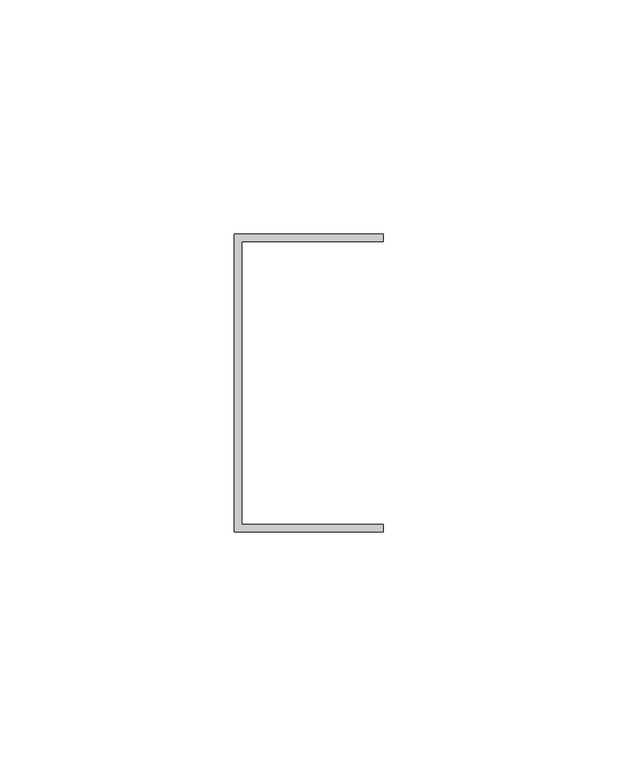
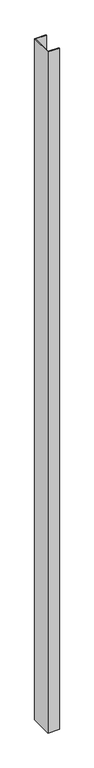
"""IFC4 building model written with IfcOpenShell, lengths in millimetres: proxy geometry, Generic Models 7:Generic Models 1:3:Generic Models 1:3 : Generic Models 7:Generic Models 1:305549:3:Generic Models 1:3:Generic Models 1:3 : Generic Models 7:Generic Models 1:305549:3 : Generic Models 7:Generic Models 1:3:Generic Models 1:3 : Generic Models 7:Generic Models 1:305549:301244:11 : Generic Models 7:Generic Models 1:3:Generic Models 1:3 : Generic Models 7:Generic Models 1:305549:3:Generic Models 1:3:Generic Models 1:3 : Generic Models 7:Generic Models 1:305549:3 : Generic Models 7:Generic Models 1:3:Generic Models 1:3 : Generic Models 7:Generic Models 1:305549:301244:308848."""

from ifc_helpers import new_model, si_unit, frame, origin, place, context, project, spatial, polyline, outline, extrude, source, transform, mapped, element, save


def generic_models_456df3e6(model_context):
    return source(origin(), model_context, "Body", "SweptSolid", [
        extrude(outline(polyline([(579161.2896713, -579013.3913842), (579193.0396713, -579013.3913842), (579193.0396713, -579014.9788842), (579162.8771713, -579014.9788842), (579162.8771713, -579075.303884), (579193.0396713, -579075.303884), (579193.0396713, -579076.891384), (579161.2896713, -579076.891384), (579161.2896713, -579013.3913842)])), frame((0.0, 0.0, 4133.81326), z_axis=(0.0, 0.0, 1.0), x_axis=(1.0, 0.0, 0.0)), (0.0, 0.0, 1.0), 2000.28674),
    ])


if __name__ == "__main__":
    model = new_model("IFC4")
    model_context = context("Model", 3, world=origin())
    ifc_project = project(units=[si_unit("LENGTHUNIT", "METRE", prefix="MILLI")], contexts=[model_context])
    site = spatial("IfcSite", under=ifc_project)
    building = spatial("IfcBuilding", under=site)
    placement = place(None, origin())
    generic_models_shape = generic_models_456df3e6(model_context)
    element("IfcBuildingElementProxy", 1, Name="Generic Models 7:Generic Models 1:3:Generic Models 1:3 : Generic Models 7:Generic Models 1:305549:3:Generic Models 1:3:Generic Models 1:3 : Generic Models 7:Generic Models 1:305549:3 : Generic Models 7:Generic Models 1:3:Generic Models 1:3 : Generic Models 7:Generic Models 1:305549:301244:11 : Generic Models 7:Generic Models 1:3:Generic Models 1:3 : Generic Models 7:Generic Models 1:305549:3:Generic Models 1:3:Generic Models 1:3 : Generic Models 7:Generic Models 1:305549:3 : Generic Models 7:Generic Models 1:3:Generic Models 1:3 : Generic Models 7:Generic Models 1:305549:301244:308848", ObjectType="Generic Models 7:Generic Models 1:3:Generic Models 1:3 : Generic Models 7:Generic Models 1:305549:3:Generic Models 1:3:Generic Models 1:3 : Generic Models 7:Generic Models 1:305549:3 : Generic Models 7:Generic Models 1:3:Generic Models 1:3 : Generic Models 7:Generic Models 1:305549:301244:11 : Generic Models 7:Generic Models 1:3:Generic Models 1:3 : Generic Models 7:Generic Models 1:305549:3:Generic Models 1:3:Generic Models 1:3 : Generic Models 7:Generic Models 1:305549:3 : Generic Models 7:Generic Models 1:3:Generic Models 1:3 : Generic Models 7:Generic Models 1:305549:301244:308848", at=placement, inside=building, context=model_context, shape_type="MappedRepresentation", body=[
        mapped(generic_models_shape, transform((0.0, 0.0, 0.0), x_axis=(1.0, 0.0, 0.0), y_axis=(0.0, 1.0, 0.0), z_axis=(0.0, 0.0, 1.0))),
    ])
    save(model, "model.ifc")

# Revit data of these elements
# Type "Generic Models 7:Generic Models 1:3:Generic Models 1:3 : Generic Models 7:Generic Models 1:305549:3:Generic Models 1:3:Generic Models 1:3 : Generic Models 7:Generic Models 1:305549:3 : Generic Models 7:Generic Models 1:3:Generic Models 1:3 : Generic Models 7:Generic Models 1:305549:301244:11 : Generic Models 7:Generic Models 1:3:Generic Models 1:3 : Generic Models 7:Generic Models 1:305549:3:Generic Models 1:3:Generic Models 1:3 : Generic Models 7:Generic Models 1:305549:3 : Generic Models 7:Generic Models 1:3:Generic Models 1:3 : Generic Models 7:Generic Models 1:305549:301244:308848"
#   NameOverride = "Generic Models 7:Generic Models 1:3:Generic Models 1:3 : Generic Models 7:Generic Models 1:305549:3:Generic Models 1:3:Generic Models 1:3 : Generic Models 7:Generic Models 1:305549:3 : Generic Models 7:Generic Models 1:3:Generic Models 1:3 : Generic Models 7:Generic Models 1:305549:301244:308848"
#   ObjectTypeOverride = "Generic Models 1:3:Generic Models 1:3 : Generic Models 7:Generic Models 1:305549:3 : Generic Models 7:Generic Models 1:3:Generic Models 1:3 : Generic Models 7:Generic Models 1:305549:301244"
#   Reference = "Generic Models 1"
#   Tag = "308848"
# Element 1 (IfcBuildingElementProxy, "Generic Models 7:Generic Models 1:3:Generic Models 1:3 : Generic Models 7:Generic Models 1:305549:3:Generic Models 1:3:Generic Models 1:3 : Generic Models 7:Generic Models 1:305549:3 : Generic Models 7:Generic Models 1:3:Generic Models 1:3 : Generic Models 7:Generic Models 1:305549:301244:11 : Generic Models 7:Generic Models 1:3:Generic Models 1:3 : Generic Models 7:Generic Models 1:305549:3:Generic Models 1:3:Generic Models 1:3 : Generic Models 7:Generic Models 1:305549:3 : Generic Models 7:Generic Models 1:3:Generic Models 1:3 : Generic Models 7:Generic Models 1:305549:301244:308848")
#   Materials on its faces: "GALVANIZED U-CHANNEL (250T125-33)"
# Materials
#   "GALVANIZED U-CHANNEL (250T125-33)": class "Unassigned", colour RGB 202 201 200, transparency 0, Keynote = "M05451300.02", Cost = 0
